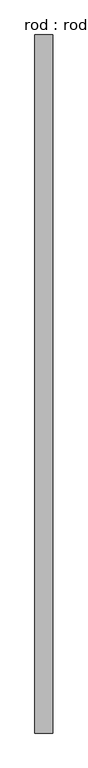
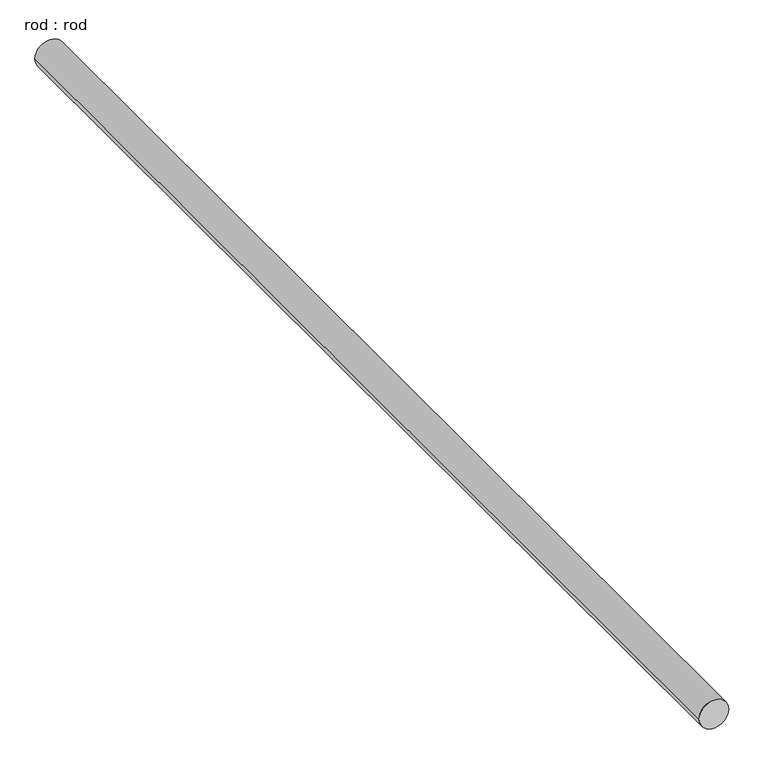
"""IFC4 building model written with IfcOpenShell, lengths in millimetres: proxy geometry, rod : rod."""

import ifcopenshell
import ifcopenshell.guid

model = None  # the IFC model being written
_history = None  # IfcOwnerHistory: only IFC2X3 demands one
_inside = {}  # id of a spatial element -> (the spatial element, [elements in it])
_under = {}  # id of a project, library or spatial element -> (it, [spatial elements below it])
_declared = {}  # id of a project -> (the project, [libraries it declares])
_typed = {}  # id of a type object -> (the type object, [elements of that type])
_made_of = {}  # id of a material, layer set ... -> (it, [elements and type objects made of it])


def new_model(schema):
    """Start an empty IFC model of exactly this schema.

    Asked for "IFC4X3", IfcOpenShell would pick the latest addendum, in which some entities
    have other attributes; the version numbers below select the first issue.
    IFC2X3 requires an IfcOwnerHistory on every rooted entity: one is made here for all.
    """
    global model, _history
    if schema == "IFC4X3":
        model = ifcopenshell.file(schema_version=(4, 3, 0, 0))
    else:
        model = ifcopenshell.file(schema=schema)
    _inside.clear()
    _under.clear()
    _declared.clear()
    _typed.clear()
    _made_of.clear()
    _history = None
    if model.schema == "IFC2X3":
        org = make("IfcOrganization", Name="unknown")
        user = make(
            "IfcPersonAndOrganization",
            ThePerson=make("IfcPerson", FamilyName="unknown"),
            TheOrganization=org,
        )
        app = make(
            "IfcApplication",
            ApplicationDeveloper=org,
            Version="unknown",
            ApplicationFullName="unknown",
            ApplicationIdentifier="unknown",
        )
        _history = make(
            "IfcOwnerHistory",
            OwningUser=user,
            OwningApplication=app,
            ChangeAction="ADDED",
            CreationDate=0,
        )
    return model


def make(cls, **values):
    """One entity of the class cls with the attributes given. An attribute that is None is left unset."""
    return model.create_entity(
        cls, **{name: value for name, value in values.items() if value is not None}
    )


def rooted(cls, **values):
    """An entity with a GlobalId (a new one), such as an element, a storey or a relation."""
    return make(cls, GlobalId=ifcopenshell.guid.new(), OwnerHistory=_history, **values)


def si_unit(unit_type, name, prefix=None):
    """IfcSIUnit, for example si_unit("LENGTHUNIT", "METRE", prefix="MILLI")."""
    return make("IfcSIUnit", UnitType=unit_type, Prefix=prefix, Name=name)


def assignment(units):
    """IfcUnitAssignment: the units of a project."""
    return None if units is None else make("IfcUnitAssignment", Units=units)


def point(xyz):
    """IfcCartesianPoint."""
    return None if xyz is None else make("IfcCartesianPoint", Coordinates=xyz)


def direction(xyz):
    """IfcDirection."""
    return None if xyz is None else make("IfcDirection", DirectionRatios=xyz)


def frame(location, z_axis=None, x_axis=None):
    """IfcAxis2Placement3D, a coordinate frame: its origin and axes. An axis left out is left unset."""
    return make(
        "IfcAxis2Placement3D",
        Location=point(location),
        Axis=direction(z_axis),
        RefDirection=direction(x_axis),
    )


def frame_2d(location, x_axis=None):
    """IfcAxis2Placement2D, a coordinate frame in the plane: its origin and x axis."""
    return make(
        "IfcAxis2Placement2D", Location=point(location), RefDirection=direction(x_axis)
    )


def origin():
    """The frame at (0, 0, 0) with its axes left unset."""
    return frame((0.0, 0.0, 0.0))


def place(relative_to, where):
    """IfcLocalPlacement: puts the frame where relative to a parent placement (None: the world)."""
    return make(
        "IfcLocalPlacement", PlacementRelTo=relative_to, RelativePlacement=where
    )


def context(
    kind, dimensions, precision=None, world=None, true_north=None, identifier=None
):
    """IfcGeometricRepresentationContext, for example the 3D "Model" context."""
    return make(
        "IfcGeometricRepresentationContext",
        ContextIdentifier=identifier,
        ContextType=kind,
        CoordinateSpaceDimension=dimensions,
        Precision=precision,
        WorldCoordinateSystem=world,
        TrueNorth=true_north,
    )


def project(units=None, contexts=None):
    """IfcProject with its units and contexts."""
    return rooted(
        "IfcProject",
        Name="project",
        RepresentationContexts=contexts,
        UnitsInContext=assignment(units),
    )


def spatial(cls, under=None, at=None, **own):
    """A site, building, storey or space (cls), placed at a placement, below another one or the project."""
    s = rooted(cls, ObjectPlacement=at, **own)
    if under is not None:
        _under.setdefault(under.id(), (under, []))[1].append(s)
    return s


def circle_curve(where, radius):
    """IfcCircle in the frame where."""
    return make("IfcCircle", Position=where, Radius=radius)


def trimmed(basis, trim1, trim2, sense, master):
    """IfcTrimmedCurve: the piece of a basis curve between two trims."""
    return make(
        "IfcTrimmedCurve",
        BasisCurve=basis,
        Trim1=trim1,
        Trim2=trim2,
        SenseAgreement=sense,
        MasterRepresentation=master,
    )


def segment(curve, same_sense, transition):
    """IfcCompositeCurveSegment."""
    return make(
        "IfcCompositeCurveSegment",
        Transition=transition,
        SameSense=same_sense,
        ParentCurve=curve,
    )


def composite_curve(segments, self_intersect=None):
    """IfcCompositeCurve: segments joined end to end."""
    return make("IfcCompositeCurve", Segments=segments, SelfIntersect=self_intersect)


def outline(outer, holes=None, kind="AREA"):
    """IfcArbitraryClosedProfileDef: a profile drawn as a closed curve; with holes, ...WithVoids."""
    if holes is None:
        return make("IfcArbitraryClosedProfileDef", ProfileType=kind, OuterCurve=outer)
    return make(
        "IfcArbitraryProfileDefWithVoids",
        ProfileType=kind,
        OuterCurve=outer,
        InnerCurves=holes,
    )


def extrude(swept, where, along, depth):
    """IfcExtrudedAreaSolid: the profile swept, set in the frame where, extruded along a direction by depth."""
    return make(
        "IfcExtrudedAreaSolid",
        SweptArea=swept,
        Position=where,
        ExtrudedDirection=direction(along),
        Depth=depth,
    )


def shape(context_of_items, identifier, shape_type, items):
    """IfcShapeRepresentation: the items that make up one representation, for example the "Body"."""
    return make(
        "IfcShapeRepresentation",
        ContextOfItems=context_of_items,
        RepresentationIdentifier=identifier,
        RepresentationType=shape_type,
        Items=items,
    )


def source(mapping_origin, context_of_items, identifier, shape_type, items):
    """IfcRepresentationMap: a shape defined once, which mapped items show again and again."""
    return make(
        "IfcRepresentationMap",
        MappingOrigin=mapping_origin,
        MappedRepresentation=shape(context_of_items, identifier, shape_type, items),
    )


def transform(
    local_origin,
    x_axis=None,
    y_axis=None,
    z_axis=None,
    scale=None,
    scale2=None,
    scale3=None,
    uniform=True,
):
    """IfcCartesianTransformationOperator3D, or its non-uniform kind. x_axis, y_axis, z_axis: its Axis1, 2, 3."""
    if uniform:
        return make(
            "IfcCartesianTransformationOperator3D",
            Axis1=direction(x_axis),
            Axis2=direction(y_axis),
            LocalOrigin=point(local_origin),
            Scale=scale,
            Axis3=direction(z_axis),
        )
    return make(
        "IfcCartesianTransformationOperator3DnonUniform",
        Axis1=direction(x_axis),
        Axis2=direction(y_axis),
        LocalOrigin=point(local_origin),
        Scale=scale,
        Axis3=direction(z_axis),
        Scale2=scale2,
        Scale3=scale3,
    )


def mapped(mapping_source, mapping_target):
    """IfcMappedItem: shows the shape of a source again, moved by a transform."""
    return make(
        "IfcMappedItem", MappingSource=mapping_source, MappingTarget=mapping_target
    )


def made_of(thing, what):
    """Note that an element or type object is made of a material, layer set ...; save() writes the relation."""
    if what is not None:
        _made_of.setdefault(what.id(), (what, []))[1].append(thing)
    return thing


def element(
    cls,
    number,
    at=None,
    inside=None,
    cuts=None,
    type_object=None,
    material=None,
    context=None,
    identifier="Body",
    shape_type=None,
    held_by="IfcProductDefinitionShape",
    body=None,
    shapes=None,
    **own,
):
    """One element of the class cls, such as IfcWall. Its Tag is "e" and its number.

    at: its placement. inside: the storey or other place that contains it. cuts: it is an
    opening in that element (IfcRelVoidsElement). A single representation is given by context,
    identifier, shape_type and body (its items); several are given by shapes. held_by: the class
    of the entity that holds the representations. save() writes the other relations.
    """
    e = rooted(cls, Tag="e%d" % number, ObjectPlacement=at, **own)
    if body is not None:
        shapes = [shape(context, identifier, shape_type, body)]
    if shapes is not None:
        e.Representation = make(held_by, Representations=shapes)
    if inside is not None:
        _inside.setdefault(inside.id(), (inside, []))[1].append(e)
    if cuts is not None:
        rooted(
            "IfcRelVoidsElement", RelatingBuildingElement=cuts, RelatedOpeningElement=e
        )
    if type_object is not None:
        _typed.setdefault(type_object.id(), (type_object, []))[1].append(e)
    return made_of(e, material)


def aggregate(whole, parts):
    """IfcRelAggregates: a whole, such as a stair, and the parts it consists of."""
    return rooted("IfcRelAggregates", RelatingObject=whole, RelatedObjects=parts)


def save(model, path):
    """Write the relations noted so far, then the file.

    IfcRelAggregates (storeys below a building ...), IfcRelContainedInSpatialStructure (elements
    in a storey), IfcRelDefinesByType, IfcRelAssociatesMaterial and IfcRelDeclares: one each for
    every whole, place, type object, material and project.
    """
    for whole, parts in _under.values():
        aggregate(whole, parts)
    for where, things in _inside.values():
        rooted(
            "IfcRelContainedInSpatialStructure",
            RelatedElements=things,
            RelatingStructure=where,
        )
    for kind, things in _typed.values():
        rooted("IfcRelDefinesByType", RelatedObjects=things, RelatingType=kind)
    for what, things in _made_of.values():
        rooted("IfcRelAssociatesMaterial", RelatedObjects=things, RelatingMaterial=what)
    for by, libraries in _declared.values():
        rooted("IfcRelDeclares", RelatingContext=by, RelatedDefinitions=libraries)
    model.write(path)


def rod_rod_699355d6(model_context):
    return source(origin(), model_context, "Body", "SweptSolid", [
        extrude(outline(composite_curve([segment(trimmed(circle_curve(frame_2d((0.0108462, 0.0)), 200.0), [point((0.0108462, 200.0))], [point((0.0108462, -200.0))], False, "CARTESIAN"), True, "CONTINUOUS"), segment(trimmed(circle_curve(frame_2d((0.0108462, 0.0)), 200.0), [point((0.0108462, -200.0))], [point((0.0108462, 200.0))], False, "CARTESIAN"), True, "CONTINUOUS")], self_intersect=False)), frame((0.0, -3657.2713847, 0.0), z_axis=(0.0, 1.0, 0.0), x_axis=(0.0, 0.0, 1.0)), (0.0, 0.0, 1.0), 15500.0),
    ])


if __name__ == "__main__":
    model = new_model("IFC4")
    model_context = context("Model", 3, world=origin())
    ifc_project = project(units=[si_unit("LENGTHUNIT", "METRE", prefix="MILLI")], contexts=[model_context])
    site = spatial("IfcSite", under=ifc_project)
    building = spatial("IfcBuilding", under=site)
    placement = place(None, origin())
    rod_rod_shape = rod_rod_699355d6(model_context)
    element("IfcBuildingElementProxy", 1, Name="rod : rod", ObjectType="rod : rod", at=placement, inside=building, context=model_context, shape_type="MappedRepresentation", body=[
        mapped(rod_rod_shape, transform((0.0, 0.0, 0.0), x_axis=(1.0, 0.0, 0.0), y_axis=(0.0, 1.0, 0.0), z_axis=(0.0, 0.0, 1.0))),
    ])
    save(model, "model.ifc")

# Revit data of these elements
# Type "rod : rod"
#   Default Elevation = 0
